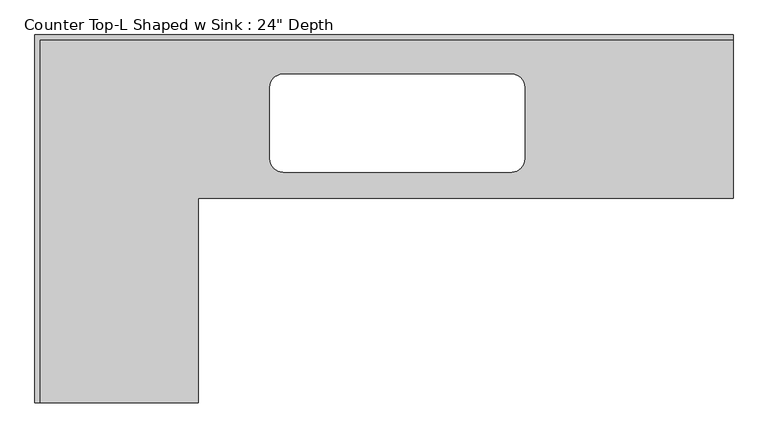
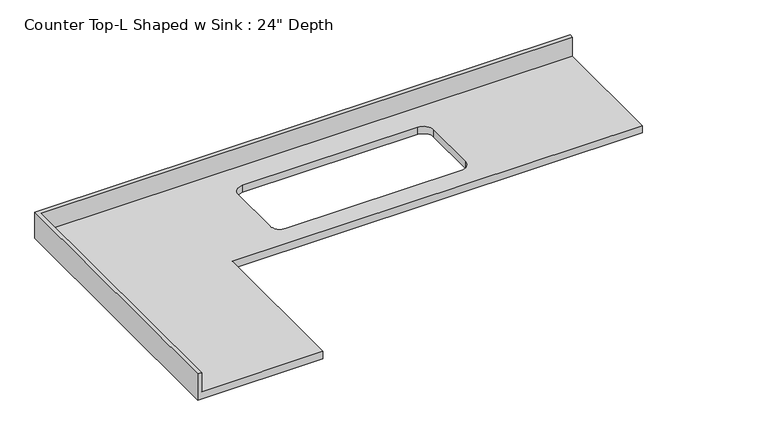
"""IFC4 building model written with IfcOpenShell, lengths in millimetres: furniture geometry."""

from ifc_helpers import new_model, si_unit, frame, origin, place, context, project, spatial, polyline, circle_curve, source, transform, mapped, element, save
from ifc_brep_helpers import plane_surface, revolved_surface, advanced_brep


def furniture_e81cc42c(model_context):
    return source(origin(), model_context, "Body", "AdvancedBrep", [
        advanced_brep(
        [(-565.4622951, -1431.2696343, 914.4), (-565.4622951, -635.0, 914.4), (1515.7502049, -635.0, 914.4), (1515.7502049, -19.05, 914.4), (-1181.4122951, -19.05, 914.4), (-1181.4122951, -1431.2696343, 914.4), (653.7377049, -152.4, 914.4), (704.5377049, -203.2, 914.4), (704.5377049, -482.6, 914.4), (653.7377049, -533.4, 914.4), (-235.2622951, -533.4, 914.4), (-286.0622951, -482.6, 914.4), (-286.0622951, -203.2, 914.4), (-235.2622951, -152.4, 914.4), (1515.7502049, 0.0, 876.3), (1515.7502049, -635.0, 876.3), (-565.4622951, -635.0, 876.3), (-565.4622951, -1431.2696343, 876.3), (-1200.4622951, -1431.2696343, 876.3), (-1200.4622951, 0.0, 876.3), (653.7377049, -152.4, 876.3), (-235.2622951, -152.4, 876.3), (-286.0622951, -203.2, 876.3), (-286.0622951, -482.6, 876.3), (-235.2622951, -533.4, 876.3), (653.7377049, -533.4, 876.3), (704.5377049, -482.6, 876.3), (704.5377049, -203.2, 876.3), (-1200.4622951, 0.0, 1016.0), (1515.7502049, 0.0, 1016.0), (-1200.4622951, -1431.2696343, 1016.0), (-1181.4122951, -1431.2696343, 1016.0), (1515.7502049, -19.05, 1016.0), (-1181.4122951, -19.05, 1016.0)],
        [
            (0, 1),
            (1, 2),
            (2, 3),
            (3, 4),
            (4, 5),
            (5, 0),
            (6, 7, circle_curve(frame((653.7377049, -203.2, 914.4), z_axis=(0.0, 0.0, -1.0), x_axis=(1.0, 0.0, 0.0)), 50.8)),
            (7, 8),
            (8, 9, circle_curve(frame((653.7377049, -482.6, 914.4), z_axis=(0.0, 0.0, -1.0), x_axis=(1.0, 0.0, 0.0)), 50.8)),
            (9, 10),
            (10, 11, circle_curve(frame((-235.2622951, -482.6, 914.4), z_axis=(0.0, 0.0, -1.0), x_axis=(1.0, 0.0, 0.0)), 50.8)),
            (11, 12),
            (12, 13, circle_curve(frame((-235.2622951, -203.2, 914.4), z_axis=(0.0, 0.0, -1.0), x_axis=(1.0, 0.0, 0.0)), 50.8)),
            (13, 6),
            (14, 15),
            (15, 16),
            (16, 17),
            (17, 18),
            (18, 19),
            (19, 14),
            (20, 21),
            (21, 22, circle_curve(frame((-235.2622951, -203.2, 876.3), z_axis=(0.0, 0.0, 1.0), x_axis=(1.0, 0.0, 0.0)), 50.8)),
            (22, 23),
            (23, 24, circle_curve(frame((-235.2622951, -482.6, 876.3), z_axis=(0.0, 0.0, 1.0), x_axis=(1.0, 0.0, 0.0)), 50.8)),
            (24, 25),
            (25, 26, circle_curve(frame((653.7377049, -482.6, 876.3), z_axis=(0.0, 0.0, 1.0), x_axis=(1.0, 0.0, 0.0)), 50.8)),
            (26, 27),
            (27, 20, circle_curve(frame((653.7377049, -203.2, 876.3), z_axis=(0.0, 0.0, 1.0), x_axis=(1.0, 0.0, 0.0)), 50.8)),
            (19, 28),
            (28, 29),
            (29, 14),
            (18, 30),
            (30, 28),
            (17, 0),
            (5, 31),
            (31, 30),
            (16, 1),
            (15, 2),
            (29, 32),
            (32, 3),
            (6, 20),
            (27, 7),
            (26, 8),
            (25, 9),
            (24, 10),
            (23, 11),
            (22, 12),
            (21, 13),
            (31, 33),
            (33, 32),
            (33, 4),
        ],
        [
            plane_surface(frame((-1200.4622951, 0.0, 914.4), z_axis=(0.0, 0.0, 1.0), x_axis=(-1.0, 0.0, 0.0))),
            plane_surface(frame((-1200.4622951, 0.0, 876.3), z_axis=(0.0, 0.0, -1.0), x_axis=(1.0, 0.0, 0.0))),
            plane_surface(frame((1515.7502049, 0.0, 914.4), z_axis=(0.0, 1.0, 0.0), x_axis=(0.0, 0.0, -1.0))),
            plane_surface(frame((-1200.4622951, 0.0, 914.4), z_axis=(-1.0, 0.0, 0.0), x_axis=(0.0, 0.0, -1.0))),
            plane_surface(frame((-1200.4622951, -1431.2696343, 914.4), z_axis=(0.0, -1.0, 0.0), x_axis=(0.0, 0.0, -1.0))),
            plane_surface(frame((-565.4622951, -1431.2696343, 914.4), z_axis=(1.0, 0.0, 0.0), x_axis=(0.0, 0.0, -1.0))),
            plane_surface(frame((-565.4622951, -635.0, 914.4), z_axis=(0.0, -1.0, 0.0), x_axis=(0.0, 0.0, -1.0))),
            plane_surface(frame((1515.7502049, -635.0, 914.4), z_axis=(1.0, 0.0, 0.0), x_axis=(0.0, 0.0, -1.0))),
            revolved_surface(polyline([(704.5377049, -203.2, 876.3), (704.5377049, -203.2, 914.4)]), (653.7377049, -203.2, 0.0), (0.0, 0.0, -1.0)),
            plane_surface(frame((704.5377049, -203.2, 914.4), z_axis=(-1.0, 0.0, 0.0), x_axis=(0.0, 0.0, -1.0))),
            revolved_surface(polyline([(704.5377049, -482.6, 876.3), (704.5377049, -482.6, 914.4)]), (653.7377049, -482.6, 0.0), (0.0, 0.0, -1.0)),
            plane_surface(frame((653.7377049, -533.4, 914.4), z_axis=(0.0, 1.0, 0.0), x_axis=(0.0, 0.0, -1.0))),
            revolved_surface(polyline([(-184.4622951, -482.6, 876.3), (-184.4622951, -482.6, 914.4)]), (-235.2622951, -482.6, 0.0), (0.0, 0.0, -1.0)),
            plane_surface(frame((-286.0622951, -482.6, 914.4), z_axis=(1.0, 0.0, 0.0), x_axis=(0.0, 0.0, -1.0))),
            revolved_surface(polyline([(-184.4622951, -203.2, 876.3), (-184.4622951, -203.2, 914.4)]), (-235.2622951, -203.2, 0.0), (0.0, 0.0, -1.0)),
            plane_surface(frame((-235.2622951, -152.4, 914.4), z_axis=(0.0, -1.0, 0.0), x_axis=(0.0, 0.0, -1.0))),
            plane_surface(frame((-1200.4622951, 0.0, 1016.0), z_axis=(0.0, 0.0, 1.0), x_axis=(0.0, -1.0, 0.0))),
            plane_surface(frame((-1200.4622951, -19.05, 1016.0), z_axis=(0.0, -1.0, 0.0), x_axis=(0.0, 0.0, -1.0))),
            plane_surface(frame((-1181.4122951, -1431.2696343, 1016.0), z_axis=(1.0, 0.0, 0.0), x_axis=(0.0, 0.0, -1.0))),
        ],
        [
            (0, [[1, 2, 3, 4, 5, 6], [7, 8, 9, 10, 11, 12, 13, 14]]),
            (1, [[15, 16, 17, 18, 19, 20], [21, 22, 23, 24, 25, 26, 27, 28]]),
            (2, [[-20, 29, 30, 31]]),
            (3, [[-19, 32, 33, -29]]),
            (4, [[-32, -18, 34, -6, 35, 36]]),
            (5, [[-1, -34, -17, 37]]),
            (6, [[-2, -37, -16, 38]]),
            (7, [[-15, -31, 39, 40, -3, -38]]),
            (8, [[-7, 41, -28, 42]]),
            (9, [[-8, -42, -27, 43]]),
            (10, [[-9, -43, -26, 44]]),
            (11, [[-10, -44, -25, 45]]),
            (12, [[-11, -45, -24, 46]]),
            (13, [[-12, -46, -23, 47]]),
            (14, [[-13, -47, -22, 48]]),
            (15, [[-14, -48, -21, -41]]),
            (16, [[-33, -36, 49, 50, -39, -30]]),
            (17, [[-40, -50, 51, -4]]),
            (18, [[-49, -35, -5, -51]]),
        ],
    ),
    ])


if __name__ == "__main__":
    model = new_model("IFC4")
    model_context = context("Model", 3, world=origin())
    ifc_project = project(units=[si_unit("LENGTHUNIT", "METRE", prefix="MILLI")], contexts=[model_context])
    site = spatial("IfcSite", under=ifc_project)
    building = spatial("IfcBuilding", under=site)
    placement = place(None, origin())
    furniture_shape = furniture_e81cc42c(model_context)
    element("IfcFurniture", 1, ObjectType="Counter Top-L Shaped w Sink : 24\" Depth", at=placement, inside=building, context=model_context, shape_type="MappedRepresentation", body=[
        mapped(furniture_shape, transform((0.0, 0.0, 0.0), x_axis=(1.0, 0.0, 0.0), y_axis=(0.0, 1.0, 0.0), z_axis=(0.0, 0.0, 1.0))),
    ])
    save(model, "model.ifc")

# Revit data of these elements
# Type "Counter Top-L Shaped w Sink : 24\" Depth"
#   Assembly Code = "C1030400"
#   Counter Thickness = 0' - 1 1/2"
#   Depth = 2' - 1"
#   Height = 3' - 0"
#   Length - Leg 1 [instance default] = 8' - 0"
#   Length - Leg 2 [instance default] = 6' - 0"
#   Sink Location [instance default] = 3' - 0"
#   Sink Location To Wall [instance default] = 0' - 6"
#   Sink Opening Depth [instance default] = 1' - 3"
#   Sink Opening Width [instance default] = 3' - 3"
#   Counter Top Material = none
# Element 1 (IfcFurniture, "Counter Top-L Shaped w Sink : 24\" Depth")
#   Length - Leg 1 = 8' - 10 15/16"
#   Length - Leg 2 = 4' - 8.3492"
#   Materials on its faces: "Counter Top"
# Materials
#   "Counter Top": class "Wood", colour RGB 226 177 128, transparency 0
